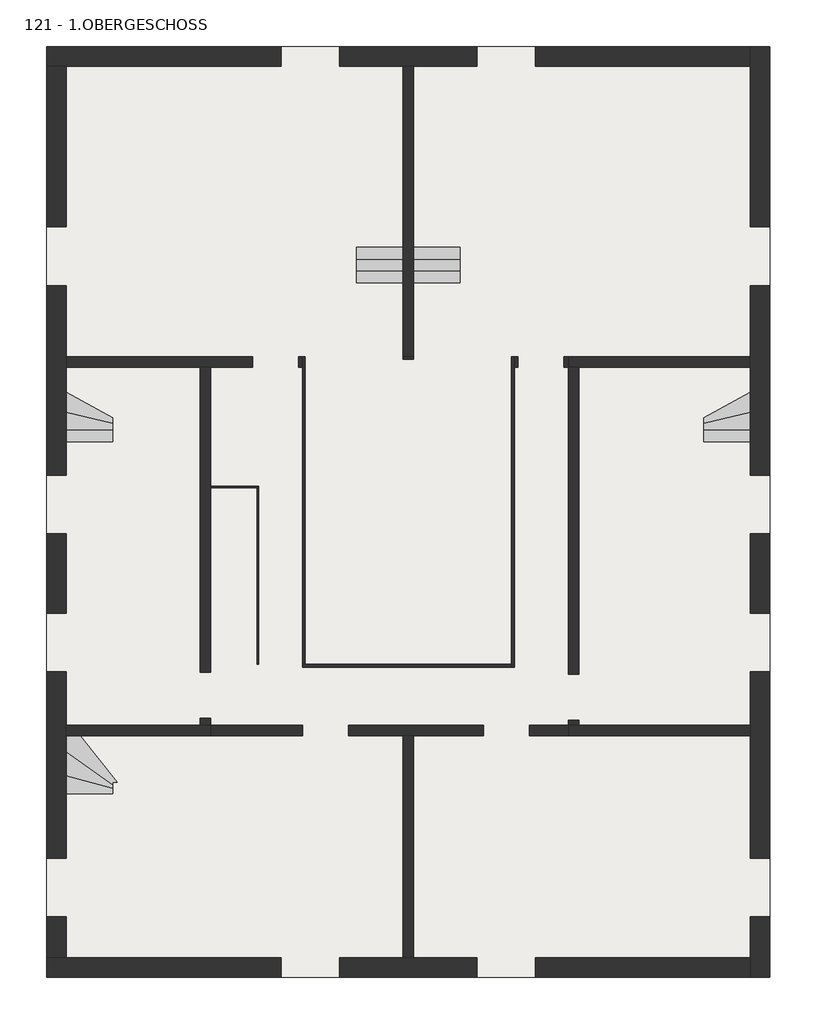
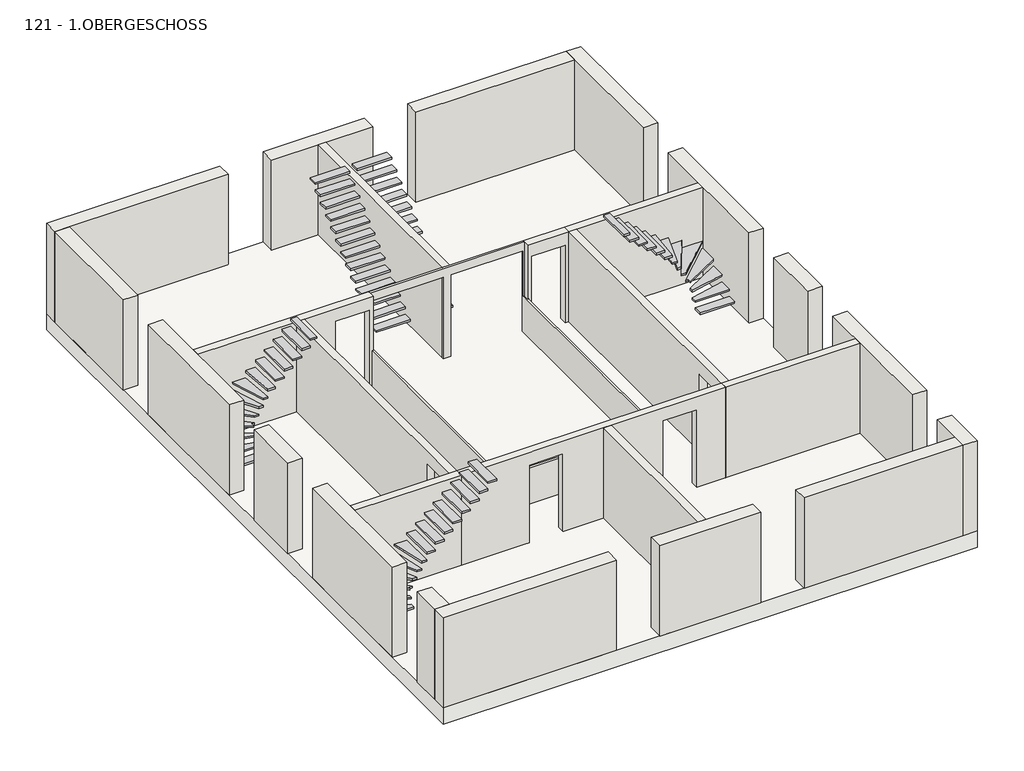
# One storey: 20 walls, 10 stairs, 1 slab.
# Revit data of these elements (continued)
# Type "  98300 :   98300"
#   Abrechnungsart = "St"
#   Allright_Bauteil_ID = "0121Tre0785065278"
#   Codetext = "TR-MASSIV-GER\\"
#   Material = "Stahlbeton"
#   Objektname = "Treppe"
#   NameOverride = " "
#   Reference = "STB-Treppe"
#   ThermalTransmittance = 0.0000 BTU/(h·ft²·°F)
#   NosingLength = 0.000 m
#   NumberOfRiser = 14
#   NumberOfTreads = 13
#   RiserHeight = 2.021 m
#   TreadLength = 2.300 m
#   IsExternal = no
#   FireExit = no
#   HandicapAccessible = no
#   HasNonSkidSurface = no
# Type "  98728 :   98728"
#   Abrechnungsart = "St"
#   Allright_Bauteil_ID = "0121Tre0785070507"
#   Material = "Stahlbeton"
#   Objektname = "Treppe"
#   NameOverride = " "
#   ThermalTransmittance = 0.0000 BTU/(h·ft²·°F)
#   NosingLength = 0.000 m
#   NumberOfRiser = 14
#   NumberOfTreads = 13
#   RiserHeight = 2.021 m
#   TreadLength = 2.300 m
#   IsExternal = no
#   FireExit = no
#   HandicapAccessible = no
#   HasNonSkidSurface = no
# Type "  99154 :   99154"
#   Abrechnungsart = "St"
#   Allright_Bauteil_ID = "0121Tre0785070829"
#   Material = "Stahlbeton"
#   Objektname = "Treppe"
#   NameOverride = " "
#   ThermalTransmittance = 0.0000 BTU/(h·ft²·°F)
#   NosingLength = 0.000 m
#   NumberOfRiser = 14
#   NumberOfTreads = 13
#   RiserHeight = 2.021 m
#   TreadLength = 2.300 m
#   IsExternal = no
#   FireExit = no
#   HandicapAccessible = no
#   HasNonSkidSurface = no
# Type "  149542 :   149542"
#   Abrechnungsart = "St"
#   Allright_Bauteil_ID = "0131Tre0659044515"
#   Material = "Stahlbeton"
#   Objektname = "Treppe"
#   NameOverride = " "
#   ThermalTransmittance = 0.0000 BTU/(h·ft²·°F)
#   NosingLength = 0.000 m
#   NumberOfRiser = 14
#   NumberOfTreads = 14
#   RiserHeight = 2.000 m
#   TreadLength = 2.300 m
#   IsExternal = no
#   FireExit = no
#   HandicapAccessible = no
#   HasNonSkidSurface = no
# Type "  150414 :   150414"
#   Abrechnungsart = "St"
#   Allright_Bauteil_ID = "0131Tre0659044575"
#   Codetext = "TR-MASSIV-GER\\"
#   Material = "Stahlbeton"
#   Objektname = "Treppe"
#   NameOverride = " "
#   Reference = "STB-Treppe"
#   ThermalTransmittance = 0.0000 BTU/(h·ft²·°F)
#   NosingLength = 0.000 m
#   NumberOfRiser = 14
#   NumberOfTreads = 13
#   RiserHeight = 2.021 m
#   TreadLength = 2.300 m
#   IsExternal = no
#   FireExit = no
#   HandicapAccessible = no
#   HasNonSkidSurface = no
# Type "  150832 :   150832"
#   Abrechnungsart = "St"
#   Allright_Bauteil_ID = "0131Tre0659044593"
#   Codetext = "TR-MASSIV-GER\\"
#   Material = "Stahlbeton"
#   Objektname = "Treppe"
#   NameOverride = " "
#   Reference = "STB-Treppe"
#   ThermalTransmittance = 0.0000 BTU/(h·ft²·°F)
#   NosingLength = 0.000 m
#   NumberOfRiser = 14
#   NumberOfTreads = 13
#   RiserHeight = 2.021 m
#   TreadLength = 2.300 m
#   IsExternal = no
#   FireExit = no
#   HandicapAccessible = no
#   HasNonSkidSurface = no
# Type "  151260 :   151260"
#   Abrechnungsart = "St"
#   Allright_Bauteil_ID = "0131Tre0659044533"
#   Material = "Stahlbeton"
#   Objektname = "Treppe"
#   NameOverride = " "
#   ThermalTransmittance = 0.0000 BTU/(h·ft²·°F)
#   NosingLength = 0.000 m
#   NumberOfRiser = 14
#   NumberOfTreads = 13
#   RiserHeight = 2.021 m
#   TreadLength = 2.300 m
#   IsExternal = no
#   FireExit = no
#   HandicapAccessible = no
#   HasNonSkidSurface = no
# Type "  151686 :   151686"
#   Abrechnungsart = "St"
#   Allright_Bauteil_ID = "0131Tre0659044570"
#   Material = "Stahlbeton"
#   Objektname = "Treppe"
#   NameOverride = " "
#   ThermalTransmittance = 0.0000 BTU/(h·ft²·°F)
#   NosingLength = 0.000 m
#   NumberOfRiser = 14
#   NumberOfTreads = 13
#   RiserHeight = 2.021 m
#   TreadLength = 2.300 m
#   IsExternal = no
#   FireExit = no
#   HandicapAccessible = no
#   HasNonSkidSurface = no
# Type " :1166"
#   Layers, outside or top first: 0.050 m "glas" (function 1)
# Type "Holzwand:1150"
#   ThermalTransmittance = 0.0000 BTU/(h·ft²·°F)
#   Combustible = no
#   Compartmentation = no
#   Layers, outside or top first: 0.200 m "holzschalung" (function 1)
# Type "Holzwand:1151"
#   ThermalTransmittance = 0.0000 BTU/(h·ft²·°F)
#   Combustible = no
#   Compartmentation = no
#   Layers, outside or top first: 0.200 m "holzschalung" (function 1)
# Type "Holzwand:1153"
#   ThermalTransmittance = 0.0000 BTU/(h·ft²·°F)
#   Combustible = no
#   Compartmentation = no
#   Layers, outside or top first: 0.200 m "holzschalung" (function 1)
# Type "Holzwand:1154"
#   ThermalTransmittance = 0.0000 BTU/(h·ft²·°F)
#   Combustible = no
#   Compartmentation = no
#   Layers, outside or top first: 0.030 m "holzschalung" (function 1)
# Type "Holzwand:1155"
#   ThermalTransmittance = 0.0000 BTU/(h·ft²·°F)
#   Combustible = no
#   Compartmentation = no
#   Layers, outside or top first: 0.030 m "holzschalung" (function 1)
# Type "Holzwand:1156"
#   ThermalTransmittance = 0.0000 BTU/(h·ft²·°F)
#   Combustible = no
#   Compartmentation = no
#   Layers, outside or top first: 0.200 m "holzschalung" (function 1)
# Type "Holzwand:1157"
#   ThermalTransmittance = 0.0000 BTU/(h·ft²·°F)
#   Combustible = no
#   Compartmentation = no
#   Layers, outside or top first: 0.200 m "holzschalung" (function 1)
# Type "Holzwand:1158"
#   ThermalTransmittance = 0.0000 BTU/(h·ft²·°F)
#   Combustible = no
#   Compartmentation = no
#   Layers, outside or top first: 0.200 m "holzschalung" (function 1)
# Type "Holzwand:1159"
#   ThermalTransmittance = 0.0000 BTU/(h·ft²·°F)
#   Combustible = no
#   Compartmentation = no
#   Layers, outside or top first: 0.200 m "holzschalung" (function 1)
# Type "Holzwand:1160"
#   ThermalTransmittance = 0.0000 BTU/(h·ft²·°F)
#   Combustible = no
#   Compartmentation = no
#   Layers, outside or top first: 0.200 m "holzschalung" (function 1)
# Type "Holzwand:1162"
#   ThermalTransmittance = 0.0000 BTU/(h·ft²·°F)
#   Combustible = no
#   Compartmentation = no
#   Layers, outside or top first: 0.200 m "holzschalung" (function 1)
# Type "Holzwand:1163"
#   ThermalTransmittance = 0.0000 BTU/(h·ft²·°F)
#   Combustible = no
#   Compartmentation = no
#   Layers, outside or top first: 0.200 m "holzschalung" (function 1)
# Type " :1167"
#   Layers, outside or top first: 0.050 m "holzschalung" (function 1)
# Type " :1168"
#   Layers, outside or top first: 0.050 m "holzschalung" (function 1)
# Type " :1169"
#   Layers, outside or top first: 0.050 m "holzschalung" (function 1)
# Type "1141 Aussenwand"
#   Layers, outside or top first: 0.380 m "holzschalung" (function 1)
# Element 1 (IfcSlab, "Holzdecke 176 : Holzdecke 176")
#   IFC Predefined Type = "FLOOR"
#   Export to IFC As = "ifcslab"
#   IfcGUID = "1_9Us2eVX4OuIZjhNyqdxW"
#   Phase Created = New Construction
#   Materials on its faces: "holzschalung"
# Element 2 (IfcStair, "  97010 :   97010")
#   IFC Predefined Type = "NOTDEFINED"
#   Export to IFC As = "ifcstair"
#   IfcGUID = "2ccaodaeb6QgHPV1d4NBnA"
#   Phase Created = New Construction
#   Materials on its faces: "weiss"
# Element 3 (IfcStair, "  97882 :   97882")
#   IFC Predefined Type = "STRAIGHT_RUN_STAIR"
#   Export to IFC As = "ifcstair"
#   IfcGUID = "1nghyUHoH9yBc_lxkBTUjw"
#   Phase Created = New Construction
#   Materials on its faces: "weiss"
# Element 4 (IfcStair, "  98300 :   98300")
#   IFC Predefined Type = "STRAIGHT_RUN_STAIR"
#   Export to IFC As = "ifcstair"
#   IfcGUID = "2AC_Gmfhz1LvYwUyPOxWan"
#   Phase Created = New Construction
#   Materials on its faces: "weiss"
# Element 5 (IfcStair, "  98728 :   98728")
#   IFC Predefined Type = "NOTDEFINED"
#   Export to IFC As = "ifcstair"
#   IfcGUID = "04Edcgbk9CPwWYiYhycXFf"
#   Phase Created = New Construction
#   Materials on its faces: "weiss"
# Element 6 (IfcStair, "  99154 :   99154")
#   IFC Predefined Type = "NOTDEFINED"
#   Export to IFC As = "ifcstair"
#   IfcGUID = "1azVXxNdn2POY9VYN93ccY"
#   Phase Created = New Construction
#   Materials on its faces: "weiss"
# Element 7 (IfcStair, "  149542 :   149542")
#   IFC Predefined Type = "NOTDEFINED"
#   Export to IFC As = "ifcstair"
#   IfcGUID = "1sH4rJKnLAFOtHPnXrLkif"
#   Phase Created = New Construction
#   Materials on its faces: "weiss"
# Element 8 (IfcStair, "  150414 :   150414")
#   IFC Predefined Type = "STRAIGHT_RUN_STAIR"
#   Export to IFC As = "ifcstair"
#   IfcGUID = "3fdccs_Mj1YAyFFpBc3gyk"
#   Phase Created = New Construction
#   Materials on its faces: "weiss"
# Element 9 (IfcStair, "  150832 :   150832")
#   IFC Predefined Type = "STRAIGHT_RUN_STAIR"
#   Export to IFC As = "ifcstair"
#   IfcGUID = "2szmEZdbD3KBDvfX1Sa6Vh"
#   Phase Created = New Construction
#   Materials on its faces: "weiss"
# Element 10 (IfcStair, "  151260 :   151260")
#   IFC Predefined Type = "NOTDEFINED"
#   Export to IFC As = "ifcstair"
#   IfcGUID = "1YKyaFTbr8YR41yGjubBsl"
#   Phase Created = New Construction
#   Materials on its faces: "weiss"
# Element 11 (IfcStair, "  151686 :   151686")
#   IFC Predefined Type = "NOTDEFINED"
#   Export to IFC As = "ifcstair"
#   IfcGUID = "2KPGRYHzzCygzBebAeLtPz"
#   Phase Created = New Construction
#   Materials on its faces: "weiss"
# Element 12 (IfcWall, " :1166")
#   Export to IFC As = "ifcwall"
#   IfcGUID = "0t2qqx1kvDZPNPdKl4bfzP"
#   NameOverride = " "
#   Abrechnungsart = "m³"
#   Allright_Bauteil_ID = "0121HWa0785064296"
#   Layer #1:Object Layer Attributes #1:Abrechnungsart = "m²"
#   Layer #1:Object Layer Attributes #1:Allright_Bauteil_ID = "0121Wa 0785064386"
#   Layer #1:Object Layer Attributes #1:Gewerk = "Zimmer- und Holzbauarbeiten"
#   Layer #1:Object Layer Attributes #1:Material = "k.Ausw."
#   Layer #1:Object Layer Attributes #1:Objektname = "Wand"
#   Layer #1:Object Layer Attributes #1:Status = "Neubau"
#   MEP Wandtyp = "HO-WA-HSW\\"
#   Objektname = "Gesamtwand"
#   built-in parameter 1001111 = 0.505 m
#   Top Offset = 0.000 m
#   Base Offset = 0.505 m
#   Unconnected Height = 2.500 m
#   wall height = 2.500 m
#   Layer #1:Object Layer Attributes #1:2D Interaktion = yes
#   Phase Created = New Construction
#   Base Constraint = 121 - 1.OBERGESCHOSS
#   Materials on its faces: "glas"
# Element 13 (IfcWall, "Holzwand:1150")
#   Export to IFC As = "ifcwall"
#   IfcGUID = "3nZ5Mon9nBjwoRgvyoor9a"
#   NameOverride = "Holzwand"
#   Abrechnungsart = "St"
#   Allright_Bauteil_ID = "0121HWa0785065367"
#   Bezeichnung = "Holzwand"
#   Layer #1:Object Layer Attributes #1:Abrechnungsart = "m²"
#   Layer #1:Object Layer Attributes #1:Allright_Bauteil_ID = "0121Wa 0785065369"
#   Layer #1:Object Layer Attributes #1:Bezeichnung = "Holzwand"
#   Layer #1:Object Layer Attributes #1:Codetext = "HO-WI-HSW\\"
#   Layer #1:Object Layer Attributes #1:Gewerk = "Zimmer- und Holzbauarbeiten"
#   Layer #1:Object Layer Attributes #1:Material = "Holz"
#   Layer #1:Object Layer Attributes #1:Objektname = "Wand"
#   Layer #1:Object Layer Attributes #1:Reference = "Holzwand"
#   Layer #1:Object Layer Attributes #1:Status = "Neubau"
#   MEP Wandtyp = "HO-WA-HSW\\"
#   Objektname = "Gesamtwand"
#   Reference = "Holzwand"
#   Status = "NEW"
#   built-in parameter 1001111 = 0.505 m
#   Top Offset = 0.000 m
#   Base Offset = 0.505 m
#   Unconnected Height = 2.500 m
#   wall height = 2.500 m
#   Layer #1:Object Layer Attributes #1:U-Wert = 0
#   Layer #1:Object Layer Attributes #1:2D Interaktion = yes
#   Layer #1:Object Layer Attributes #1:Außenbauteil = no
#   Layer #1:Object Layer Attributes #1:Brandabschnittsdefinierendes Bauteil = no
#   Layer #1:Object Layer Attributes #1:Brennbares Material = no
#   Layer #1:Object Layer Attributes #1:Raumhohe Wand = yes
#   Layer #1:Object Layer Attributes #1:Tragendes Bauteil = yes
#   ExtendToStructure = yes
#   IsExternal = no
#   LoadBearing = yes
#   Phase Created = New Construction
#   Base Constraint = 121 - 1.OBERGESCHOSS
#   Materials on its faces: "holzschalung"
# Element 14 (IfcWall, "Holzwand:1151")
#   Export to IFC As = "ifcwall"
#   IfcGUID = "3jE1E$NFj7vAP$vn70kdrt"
#   NameOverride = "Holzwand"
#   Abrechnungsart = "St"
#   Allright_Bauteil_ID = "0121HWa0785066899"
#   Bezeichnung = "Holzwand"
#   Layer #1:Object Layer Attributes #1:Abrechnungsart = "m²"
#   Layer #1:Object Layer Attributes #1:Allright_Bauteil_ID = "0121Wa 0785066901"
#   Layer #1:Object Layer Attributes #1:Bezeichnung = "Holzwand"
#   Layer #1:Object Layer Attributes #1:Codetext = "HO-WI-HSW\\"
#   Layer #1:Object Layer Attributes #1:Gewerk = "Zimmer- und Holzbauarbeiten"
#   Layer #1:Object Layer Attributes #1:Material = "Holz"
#   Layer #1:Object Layer Attributes #1:Objektname = "Wand"
#   Layer #1:Object Layer Attributes #1:Reference = "Holzwand"
#   Layer #1:Object Layer Attributes #1:Status = "Neubau"
#   MEP Wandtyp = "HO-WA-HSW\\"
#   Objektname = "Gesamtwand"
#   Reference = "Holzwand"
#   Status = "NEW"
#   built-in parameter 1001111 = 0.505 m
#   Top Offset = 0.000 m
#   Base Offset = 0.505 m
#   Unconnected Height = 2.500 m
#   wall height = 2.500 m
#   Layer #1:Object Layer Attributes #1:U-Wert = 0
#   Layer #1:Object Layer Attributes #1:2D Interaktion = yes
#   Layer #1:Object Layer Attributes #1:Außenbauteil = no
#   Layer #1:Object Layer Attributes #1:Brandabschnittsdefinierendes Bauteil = no
#   Layer #1:Object Layer Attributes #1:Brennbares Material = no
#   Layer #1:Object Layer Attributes #1:Raumhohe Wand = yes
#   Layer #1:Object Layer Attributes #1:Tragendes Bauteil = yes
#   ExtendToStructure = yes
#   IsExternal = no
#   LoadBearing = yes
#   Phase Created = New Construction
#   Base Constraint = 121 - 1.OBERGESCHOSS
#   Materials on its faces: "holzschalung"
# Element 15 (IfcWall, "Holzwand:1153")
#   Export to IFC As = "ifcwall"
#   IfcGUID = "1Zhxv5EALB9e6_$pCtUEXg"
#   NameOverride = "Holzwand"
#   Abrechnungsart = "St"
#   Allright_Bauteil_ID = "0121HWa0785065540"
#   Bezeichnung = "Holzwand"
#   Layer #1:Object Layer Attributes #1:Abrechnungsart = "m²"
#   Layer #1:Object Layer Attributes #1:Allright_Bauteil_ID = "0121Wa 0785065541"
#   Layer #1:Object Layer Attributes #1:Bezeichnung = "Holzwand"
#   Layer #1:Object Layer Attributes #1:Codetext = "HO-WI-HSW\\"
#   Layer #1:Object Layer Attributes #1:Gewerk = "Zimmer- und Holzbauarbeiten"
#   Layer #1:Object Layer Attributes #1:Material = "Holz"
#   Layer #1:Object Layer Attributes #1:Objektname = "Wand"
#   Layer #1:Object Layer Attributes #1:Reference = "Holzwand"
#   Layer #1:Object Layer Attributes #1:Status = "Neubau"
#   MEP Wandtyp = "HO-WA-HSW\\"
#   Objektname = "Gesamtwand"
#   Reference = "Holzwand"
#   Status = "NEW"
#   built-in parameter 1001111 = 0.505 m
#   Top Offset = 0.000 m
#   Base Offset = 0.505 m
#   Unconnected Height = 2.500 m
#   wall height = 2.500 m
#   Layer #1:Object Layer Attributes #1:U-Wert = 0
#   Layer #1:Object Layer Attributes #1:2D Interaktion = yes
#   Layer #1:Object Layer Attributes #1:Außenbauteil = no
#   Layer #1:Object Layer Attributes #1:Brandabschnittsdefinierendes Bauteil = no
#   Layer #1:Object Layer Attributes #1:Brennbares Material = no
#   Layer #1:Object Layer Attributes #1:Raumhohe Wand = yes
#   Layer #1:Object Layer Attributes #1:Tragendes Bauteil = yes
#   ExtendToStructure = yes
#   IsExternal = no
#   LoadBearing = yes
#   Phase Created = New Construction
#   Base Constraint = 121 - 1.OBERGESCHOSS
#   Materials on its faces: "holzschalung"
# Element 16 (IfcWall, "Holzwand:1154")
#   Export to IFC As = "ifcwall"
#   IfcGUID = "2MsVq3EJn0K8wHdQ6uoxnd"
#   NameOverride = "Holzwand"
#   Abrechnungsart = "St"
#   Allright_Bauteil_ID = "0121HWa0785067355"
#   Bezeichnung = "Holzwand"
#   Layer #1:Object Layer Attributes #1:Abrechnungsart = "m²"
#   Layer #1:Object Layer Attributes #1:Allright_Bauteil_ID = "0121Wa 0785067356"
#   Layer #1:Object Layer Attributes #1:Codetext = "HO-WI-HSW\\"
#   Layer #1:Object Layer Attributes #1:Gewerk = "Zimmer- und Holzbauarbeiten"
#   Layer #1:Object Layer Attributes #1:Material = "Holz"
#   Layer #1:Object Layer Attributes #1:Objektname = "Wand"
#   Layer #1:Object Layer Attributes #1:Reference = "Holzwand"
#   Layer #1:Object Layer Attributes #1:Status = "Neubau"
#   MEP Wandtyp = "HO-WA-HSW\\"
#   Objektname = "Gesamtwand"
#   Reference = "Holzwand"
#   Status = "NEW"
#   built-in parameter 1001111 = 0.505 m
#   Top Offset = 0.000 m
#   Base Offset = 0.505 m
#   Unconnected Height = 1.000 m
#   wall height = 1.000 m
#   Layer #1:Object Layer Attributes #1:U-Wert = 0
#   Layer #1:Object Layer Attributes #1:2D Interaktion = yes
#   Layer #1:Object Layer Attributes #1:Außenbauteil = no
#   Layer #1:Object Layer Attributes #1:Brandabschnittsdefinierendes Bauteil = no
#   Layer #1:Object Layer Attributes #1:Brennbares Material = no
#   Layer #1:Object Layer Attributes #1:Raumhohe Wand = yes
#   ExtendToStructure = yes
#   IsExternal = no
#   LoadBearing = yes
#   Phase Created = New Construction
#   Base Constraint = 121 - 1.OBERGESCHOSS
#   Materials on its faces: "holzschalung"
# Element 17 (IfcWall, "Holzwand:1155")
#   Export to IFC As = "ifcwall"
#   IfcGUID = "1F_ySrDsP9oP3MqXymSTVO"
#   NameOverride = "Holzwand"
#   Abrechnungsart = "St"
#   Allright_Bauteil_ID = "0121HWa0785067347"
#   Bezeichnung = "Holzwand"
#   Layer #1:Object Layer Attributes #1:Abrechnungsart = "m²"
#   Layer #1:Object Layer Attributes #1:Allright_Bauteil_ID = "0121Wa 0785067348"
#   Layer #1:Object Layer Attributes #1:Codetext = "HO-WI-HSW\\"
#   Layer #1:Object Layer Attributes #1:Gewerk = "Zimmer- und Holzbauarbeiten"
#   Layer #1:Object Layer Attributes #1:Material = "Holz"
#   Layer #1:Object Layer Attributes #1:Objektname = "Wand"
#   Layer #1:Object Layer Attributes #1:Reference = "Holzwand"
#   Layer #1:Object Layer Attributes #1:Status = "Neubau"
#   MEP Wandtyp = "HO-WA-HSW\\"
#   Objektname = "Gesamtwand"
#   Reference = "Holzwand"
#   Status = "NEW"
#   built-in parameter 1001111 = 0.505 m
#   Top Offset = 0.000 m
#   Base Offset = 0.505 m
#   Unconnected Height = 1.000 m
#   wall height = 1.000 m
#   Layer #1:Object Layer Attributes #1:U-Wert = 0
#   Layer #1:Object Layer Attributes #1:2D Interaktion = yes
#   Layer #1:Object Layer Attributes #1:Außenbauteil = no
#   Layer #1:Object Layer Attributes #1:Brandabschnittsdefinierendes Bauteil = no
#   Layer #1:Object Layer Attributes #1:Brennbares Material = no
#   Layer #1:Object Layer Attributes #1:Raumhohe Wand = yes
#   ExtendToStructure = yes
#   IsExternal = no
#   LoadBearing = yes
#   Phase Created = New Construction
#   Base Constraint = 121 - 1.OBERGESCHOSS
#   Materials on its faces: "holzschalung"
# Element 18 (IfcWall, "Holzwand:1156")
#   Export to IFC As = "ifcwall"
#   IfcGUID = "0gtwZwppj1pObqyI7HY41_"
#   NameOverride = "Holzwand"
#   Abrechnungsart = "St"
#   Allright_Bauteil_ID = "0121HWa0785064323"
#   Bezeichnung = "Holzwand"
#   Layer #1:Object Layer Attributes #1:Abrechnungsart = "m²"
#   Layer #1:Object Layer Attributes #1:Allright_Bauteil_ID = "0121Wa 0785064369"
#   Layer #1:Object Layer Attributes #1:Bezeichnung = "Holzwand"
#   Layer #1:Object Layer Attributes #1:Codetext = "HO-WI-HSW\\"
#   Layer #1:Object Layer Attributes #1:Gewerk = "Zimmer- und Holzbauarbeiten"
#   Layer #1:Object Layer Attributes #1:Material = "Holz"
#   Layer #1:Object Layer Attributes #1:Objektname = "Wand"
#   Layer #1:Object Layer Attributes #1:Reference = "Holzwand"
#   Layer #1:Object Layer Attributes #1:Status = "Neubau"
#   MEP Wandtyp = "HO-WA-HSW\\"
#   Objektname = "Gesamtwand"
#   Reference = "Holzwand"
#   Status = "NEW"
#   built-in parameter 1001111 = 0.505 m
#   Top Offset = 0.000 m
#   Base Offset = 0.505 m
#   Unconnected Height = 2.500 m
#   wall height = 2.500 m
#   Layer #1:Object Layer Attributes #1:U-Wert = 0
#   Layer #1:Object Layer Attributes #1:2D Interaktion = yes
#   Layer #1:Object Layer Attributes #1:Außenbauteil = no
#   Layer #1:Object Layer Attributes #1:Brandabschnittsdefinierendes Bauteil = no
#   Layer #1:Object Layer Attributes #1:Brennbares Material = no
#   Layer #1:Object Layer Attributes #1:Raumhohe Wand = yes
#   Layer #1:Object Layer Attributes #1:Tragendes Bauteil = yes
#   ExtendToStructure = yes
#   IsExternal = no
#   LoadBearing = yes
#   Phase Created = New Construction
#   Base Constraint = 121 - 1.OBERGESCHOSS
#   Materials on its faces: "holzschalung"
# Element 19 (IfcWall, "Holzwand:1157")
#   Export to IFC As = "ifcwall"
#   IfcGUID = "0tY6$O1l121AktLhYSWZjf"
#   NameOverride = "Holzwand"
#   Abrechnungsart = "St"
#   Allright_Bauteil_ID = "0121HWa0785064381"
#   Bezeichnung = "Holzwand"
#   Layer #1:Object Layer Attributes #1:Abrechnungsart = "m²"
#   Layer #1:Object Layer Attributes #1:Allright_Bauteil_ID = "0121Wa 0785064384"
#   Layer #1:Object Layer Attributes #1:Bezeichnung = "Holzwand"
#   Layer #1:Object Layer Attributes #1:Codetext = "HO-WI-HSW\\"
#   Layer #1:Object Layer Attributes #1:Gewerk = "Zimmer- und Holzbauarbeiten"
#   Layer #1:Object Layer Attributes #1:Material = "Holz"
#   Layer #1:Object Layer Attributes #1:Objektname = "Wand"
#   Layer #1:Object Layer Attributes #1:Reference = "Holzwand"
#   Layer #1:Object Layer Attributes #1:Status = "Neubau"
#   MEP Wandtyp = "HO-WA-HSW\\"
#   Objektname = "Gesamtwand"
#   Reference = "Holzwand"
#   Status = "NEW"
#   built-in parameter 1001111 = 0.505 m
#   Top Offset = 0.000 m
#   Base Offset = 0.505 m
#   Unconnected Height = 2.500 m
#   wall height = 2.500 m
#   Layer #1:Object Layer Attributes #1:U-Wert = 0
#   Layer #1:Object Layer Attributes #1:2D Interaktion = yes
#   Layer #1:Object Layer Attributes #1:Außenbauteil = no
#   Layer #1:Object Layer Attributes #1:Brandabschnittsdefinierendes Bauteil = no
#   Layer #1:Object Layer Attributes #1:Brennbares Material = no
#   Layer #1:Object Layer Attributes #1:Raumhohe Wand = yes
#   Layer #1:Object Layer Attributes #1:Tragendes Bauteil = yes
#   ExtendToStructure = yes
#   IsExternal = no
#   LoadBearing = yes
#   Phase Created = New Construction
#   Base Constraint = 121 - 1.OBERGESCHOSS
#   Materials on its faces: "holzschalung"
# Element 20 (IfcWall, "Holzwand:1158")
#   Export to IFC As = "ifcwall"
#   IfcGUID = "2Mr8L52dj4iP8MoJTiOa9p"
#   NameOverride = "Holzwand"
#   Abrechnungsart = "St"
#   Allright_Bauteil_ID = "0121HWa0785069286"
#   Bezeichnung = "Holzwand"
#   Layer #1:Object Layer Attributes #1:Abrechnungsart = "m²"
#   Layer #1:Object Layer Attributes #1:Allright_Bauteil_ID = "0121Wa 0785069294"
#   Layer #1:Object Layer Attributes #1:Bezeichnung = "Holzwand"
#   Layer #1:Object Layer Attributes #1:Codetext = "HO-WI-HSW\\"
#   Layer #1:Object Layer Attributes #1:Gewerk = "Zimmer- und Holzbauarbeiten"
#   Layer #1:Object Layer Attributes #1:Material = "Holz"
#   Layer #1:Object Layer Attributes #1:Objektname = "Wand"
#   Layer #1:Object Layer Attributes #1:Reference = "Holzwand"
#   Layer #1:Object Layer Attributes #1:Status = "Neubau"
#   MEP Wandtyp = "HO-WA-HSW\\"
#   Objektname = "Gesamtwand"
#   Reference = "Holzwand"
#   Status = "NEW"
#   built-in parameter 1001111 = 0.505 m
#   Top Offset = 0.000 m
#   Base Offset = 0.505 m
#   Unconnected Height = 2.500 m
#   wall height = 2.500 m
#   Layer #1:Object Layer Attributes #1:U-Wert = 0
#   Layer #1:Object Layer Attributes #1:2D Interaktion = yes
#   Layer #1:Object Layer Attributes #1:Außenbauteil = no
#   Layer #1:Object Layer Attributes #1:Brandabschnittsdefinierendes Bauteil = no
#   Layer #1:Object Layer Attributes #1:Brennbares Material = no
#   Layer #1:Object Layer Attributes #1:Raumhohe Wand = yes
#   Layer #1:Object Layer Attributes #1:Tragendes Bauteil = yes
#   ExtendToStructure = yes
#   IsExternal = no
#   LoadBearing = yes
#   Phase Created = New Construction
#   Base Constraint = 121 - 1.OBERGESCHOSS
#   Materials on its faces: "holzschalung"
# Element 21 (IfcWall, "Holzwand:1159")
#   Export to IFC As = "ifcwall"
#   IfcGUID = "36leNf4gL9OB_v358ffY76"
#   NameOverride = "Holzwand"
#   Abrechnungsart = "St"
#   Allright_Bauteil_ID = "0121HWa0785064324"
#   Bezeichnung = "Holzwand"
#   Layer #1:Object Layer Attributes #1:Abrechnungsart = "m²"
#   Layer #1:Object Layer Attributes #1:Allright_Bauteil_ID = "0121Wa 0785064395"
#   Layer #1:Object Layer Attributes #1:Bezeichnung = "Holzwand"
#   Layer #1:Object Layer Attributes #1:Codetext = "HO-WI-HSW\\"
#   Layer #1:Object Layer Attributes #1:Gewerk = "Zimmer- und Holzbauarbeiten"
#   Layer #1:Object Layer Attributes #1:Material = "Holz"
#   Layer #1:Object Layer Attributes #1:Objektname = "Wand"
#   Layer #1:Object Layer Attributes #1:Reference = "Holzwand"
#   Layer #1:Object Layer Attributes #1:Status = "Neubau"
#   MEP Wandtyp = "HO-WA-HSW\\"
#   Objektname = "Gesamtwand"
#   Reference = "Holzwand"
#   Status = "NEW"
#   built-in parameter 1001111 = 0.505 m
#   Top Offset = 0.000 m
#   Base Offset = 0.505 m
#   Unconnected Height = 2.500 m
#   wall height = 2.500 m
#   Layer #1:Object Layer Attributes #1:U-Wert = 0
#   Layer #1:Object Layer Attributes #1:2D Interaktion = yes
#   Layer #1:Object Layer Attributes #1:Außenbauteil = no
#   Layer #1:Object Layer Attributes #1:Brandabschnittsdefinierendes Bauteil = no
#   Layer #1:Object Layer Attributes #1:Brennbares Material = no
#   Layer #1:Object Layer Attributes #1:Raumhohe Wand = yes
#   Layer #1:Object Layer Attributes #1:Tragendes Bauteil = yes
#   ExtendToStructure = yes
#   IsExternal = no
#   LoadBearing = yes
#   Phase Created = New Construction
#   Base Constraint = 121 - 1.OBERGESCHOSS
#   Materials on its faces: "holzschalung"
# Element 22 (IfcWall, "Holzwand:1160")
#   Export to IFC As = "ifcwall"
#   IfcGUID = "3kHHpx_NTE_9JnfL3dFkYB"
#   NameOverride = "Holzwand"
#   Abrechnungsart = "St"
#   Allright_Bauteil_ID = "0121HWa0785064389"
#   Bezeichnung = "Holzwand"
#   Layer #1:Object Layer Attributes #1:Abrechnungsart = "m²"
#   Layer #1:Object Layer Attributes #1:Allright_Bauteil_ID = "0121Wa 0785064393"
#   Layer #1:Object Layer Attributes #1:Bezeichnung = "Holzwand"
#   Layer #1:Object Layer Attributes #1:Codetext = "HO-WI-HSW\\"
#   Layer #1:Object Layer Attributes #1:Gewerk = "Zimmer- und Holzbauarbeiten"
#   Layer #1:Object Layer Attributes #1:Material = "Holz"
#   Layer #1:Object Layer Attributes #1:Objektname = "Wand"
#   Layer #1:Object Layer Attributes #1:Reference = "Holzwand"
#   Layer #1:Object Layer Attributes #1:Status = "Neubau"
#   MEP Wandtyp = "HO-WA-HSW\\"
#   Objektname = "Gesamtwand"
#   Reference = "Holzwand"
#   Status = "NEW"
#   built-in parameter 1001111 = 0.505 m
#   Top Offset = 0.000 m
#   Base Offset = 0.505 m
#   Unconnected Height = 2.500 m
#   wall height = 2.500 m
#   Layer #1:Object Layer Attributes #1:U-Wert = 0
#   Layer #1:Object Layer Attributes #1:2D Interaktion = yes
#   Layer #1:Object Layer Attributes #1:Außenbauteil = no
#   Layer #1:Object Layer Attributes #1:Brandabschnittsdefinierendes Bauteil = no
#   Layer #1:Object Layer Attributes #1:Brennbares Material = no
#   Layer #1:Object Layer Attributes #1:Raumhohe Wand = yes
#   Layer #1:Object Layer Attributes #1:Tragendes Bauteil = yes
#   ExtendToStructure = yes
#   IsExternal = no
#   LoadBearing = yes
#   Phase Created = New Construction
#   Base Constraint = 121 - 1.OBERGESCHOSS
#   Materials on its faces: "holzschalung"
# Element 23 (IfcWall, "Holzwand:1162")
#   Export to IFC As = "ifcwall"
#   IfcGUID = "26lQuimMP00PZvPhbBRI2R"
#   NameOverride = "Holzwand"
#   Abrechnungsart = "St"
#   Allright_Bauteil_ID = "0121HWa0785065329"
#   Bezeichnung = "Holzwand"
#   Layer #1:Object Layer Attributes #1:Abrechnungsart = "m²"
#   Layer #1:Object Layer Attributes #1:Allright_Bauteil_ID = "0121Wa 0785065331"
#   Layer #1:Object Layer Attributes #1:Bezeichnung = "Holzwand"
#   Layer #1:Object Layer Attributes #1:Codetext = "HO-WI-HSW\\"
#   Layer #1:Object Layer Attributes #1:Gewerk = "Zimmer- und Holzbauarbeiten"
#   Layer #1:Object Layer Attributes #1:Material = "Holz"
#   Layer #1:Object Layer Attributes #1:Objektname = "Wand"
#   Layer #1:Object Layer Attributes #1:Reference = "Holzwand"
#   Layer #1:Object Layer Attributes #1:Status = "Neubau"
#   MEP Wandtyp = "HO-WA-HSW\\"
#   Objektname = "Gesamtwand"
#   Reference = "Holzwand"
#   Status = "NEW"
#   built-in parameter 1001111 = 0.505 m
#   Top Offset = 0.000 m
#   Base Offset = 0.505 m
#   Unconnected Height = 2.500 m
#   wall height = 2.500 m
#   Layer #1:Object Layer Attributes #1:U-Wert = 0
#   Layer #1:Object Layer Attributes #1:2D Interaktion = yes
#   Layer #1:Object Layer Attributes #1:Außenbauteil = no
#   Layer #1:Object Layer Attributes #1:Brandabschnittsdefinierendes Bauteil = no
#   Layer #1:Object Layer Attributes #1:Brennbares Material = no
#   Layer #1:Object Layer Attributes #1:Raumhohe Wand = yes
#   Layer #1:Object Layer Attributes #1:Tragendes Bauteil = yes
#   ExtendToStructure = yes
#   IsExternal = no
#   LoadBearing = yes
#   Phase Created = New Construction
#   Base Constraint = 121 - 1.OBERGESCHOSS
#   Materials on its faces: "holzschalung"
# Element 24 (IfcWall, "Holzwand:1163")
#   Export to IFC As = "ifcwall"
#   IfcGUID = "3atU$IMTH8YP$GZozT8ehc"
#   NameOverride = "Holzwand"
#   Abrechnungsart = "St"
#   Allright_Bauteil_ID = "0121HWa0785064334"
#   Bezeichnung = "Holzwand"
#   Layer #1:Object Layer Attributes #1:Abrechnungsart = "m²"
#   Layer #1:Object Layer Attributes #1:Allright_Bauteil_ID = "0121Wa 0785064371"
#   Layer #1:Object Layer Attributes #1:Bezeichnung = "Holzwand"
#   Layer #1:Object Layer Attributes #1:Codetext = "HO-WI-HSW\\"
#   Layer #1:Object Layer Attributes #1:Gewerk = "Zimmer- und Holzbauarbeiten"
#   Layer #1:Object Layer Attributes #1:Material = "Holz"
#   Layer #1:Object Layer Attributes #1:Objektname = "Wand"
#   Layer #1:Object Layer Attributes #1:Reference = "Holzwand"
#   Layer #1:Object Layer Attributes #1:Status = "Neubau"
#   MEP Wandtyp = "HO-WA-HSW\\"
#   Objektname = "Gesamtwand"
#   Reference = "Holzwand"
#   Status = "NEW"
#   built-in parameter 1001111 = 0.505 m
#   Top Offset = 0.000 m
#   Base Offset = 0.505 m
#   Unconnected Height = 2.500 m
#   wall height = 2.500 m
#   Layer #1:Object Layer Attributes #1:U-Wert = 0
#   Layer #1:Object Layer Attributes #1:2D Interaktion = yes
#   Layer #1:Object Layer Attributes #1:Außenbauteil = no
#   Layer #1:Object Layer Attributes #1:Brandabschnittsdefinierendes Bauteil = no
#   Layer #1:Object Layer Attributes #1:Brennbares Material = no
#   Layer #1:Object Layer Attributes #1:Raumhohe Wand = yes
#   Layer #1:Object Layer Attributes #1:Tragendes Bauteil = yes
#   ExtendToStructure = yes
#   IsExternal = no
#   LoadBearing = yes
#   Phase Created = New Construction
#   Base Constraint = 121 - 1.OBERGESCHOSS
#   Materials on its faces: "holzschalung"
# Element 25 (IfcWall, " :1167")
#   Export to IFC As = "ifcwall"
#   IfcGUID = "35Iolt9MTFw82QPYPk5JvU"
#   NameOverride = " "
#   Abrechnungsart = "m³"
#   Allright_Bauteil_ID = "0121HWa0785064294"
#   Layer #1:Object Layer Attributes #1:Abrechnungsart = "m²"
#   Layer #1:Object Layer Attributes #1:Allright_Bauteil_ID = "0121Wa 0785064340"
#   Layer #1:Object Layer Attributes #1:Gewerk = "Zimmer- und Holzbauarbeiten"
#   Layer #1:Object Layer Attributes #1:Material = "k.Ausw."
#   Layer #1:Object Layer Attributes #1:Objektname = "Wand"
#   Layer #1:Object Layer Attributes #1:Status = "Neubau"
#   MEP Wandtyp = "HO-WA-HSW\\"
#   Objektname = "Gesamtwand"
#   built-in parameter 1001111 = 0.505 m
#   Top Offset = 0.000 m
#   Base Offset = 0.505 m
#   Unconnected Height = 1.000 m
#   wall height = 1.000 m
#   Layer #1:Object Layer Attributes #1:2D Interaktion = yes
#   Layer #1:Object Layer Attributes #1:Tragendes Bauteil = no
#   Phase Created = New Construction
#   Base Constraint = 121 - 1.OBERGESCHOSS
#   Materials on its faces: "holzschalung", "glas"
# Element 26 (IfcWall, " :1168")
#   Export to IFC As = "ifcwall"
#   IfcGUID = "21NDiotIv7sAO2c5Bbio25"
#   NameOverride = " "
#   Abrechnungsart = "m³"
#   Allright_Bauteil_ID = "0121HWa0785064290"
#   Layer #1:Object Layer Attributes #1:Abrechnungsart = "m²"
#   Layer #1:Object Layer Attributes #1:Allright_Bauteil_ID = "0121Wa 0785064348"
#   Layer #1:Object Layer Attributes #1:Gewerk = "Zimmer- und Holzbauarbeiten"
#   Layer #1:Object Layer Attributes #1:Material = "k.Ausw."
#   Layer #1:Object Layer Attributes #1:Objektname = "Wand"
#   Layer #1:Object Layer Attributes #1:Status = "Neubau"
#   MEP Wandtyp = "HO-WA-HSW\\"
#   Objektname = "Gesamtwand"
#   built-in parameter 1001111 = 0.505 m
#   Top Offset = 0.000 m
#   Base Offset = 0.505 m
#   Unconnected Height = 1.000 m
#   wall height = 1.000 m
#   Layer #1:Object Layer Attributes #1:2D Interaktion = yes
#   Layer #1:Object Layer Attributes #1:Tragendes Bauteil = no
#   Phase Created = New Construction
#   Base Constraint = 121 - 1.OBERGESCHOSS
#   Materials on its faces: "holzschalung"
# Element 27 (IfcWall, " :1169")
#   Export to IFC As = "ifcwall"
#   IfcGUID = "2aL_F8tebFMgUeEEKPH5KO"
#   NameOverride = " "
#   Abrechnungsart = "m³"
#   Allright_Bauteil_ID = "0121HWa0785064292"
#   Layer #1:Object Layer Attributes #1:Abrechnungsart = "m²"
#   Layer #1:Object Layer Attributes #1:Allright_Bauteil_ID = "0121Wa 0785064346"
#   Layer #1:Object Layer Attributes #1:Gewerk = "Zimmer- und Holzbauarbeiten"
#   Layer #1:Object Layer Attributes #1:Material = "k.Ausw."
#   Layer #1:Object Layer Attributes #1:Objektname = "Wand"
#   Layer #1:Object Layer Attributes #1:Status = "Neubau"
#   MEP Wandtyp = "HO-WA-HSW\\"
#   Objektname = "Gesamtwand"
#   built-in parameter 1001111 = 0.505 m
#   Top Offset = 0.000 m
#   Base Offset = 0.505 m
#   Unconnected Height = 1.000 m
#   wall height = 1.000 m
#   Layer #1:Object Layer Attributes #1:2D Interaktion = yes
#   Layer #1:Object Layer Attributes #1:Tragendes Bauteil = no
#   Phase Created = New Construction
#   Base Constraint = 121 - 1.OBERGESCHOSS
#   Materials on its faces: "holzschalung", "glas"
# Element 28 (IfcWall, "1141 Aussenwand")
#   Export to IFC As = "ifcwall"
#   IfcGUID = "2CeDj8YZTCPx$yj4WDVOez"
#   NameOverride = " "
#   Abrechnungsart = "m³"
#   Allright_Bauteil_ID = "0121HWa0785064286"
#   Layer #1:Object Layer Attributes #1:Abrechnungsart = "m²"
#   Layer #1:Object Layer Attributes #1:Allright_Bauteil_ID = "0121Wa 0785064367"
#   Layer #1:Object Layer Attributes #1:Gewerk = "Zimmer- und Holzbauarbeiten"
#   Layer #1:Object Layer Attributes #1:Material = "k.Ausw."
#   Layer #1:Object Layer Attributes #1:Objektname = "Wand"
#   Layer #1:Object Layer Attributes #1:Status = "Neubau"
#   MEP Wandtyp = "HO-WA-HSW\\"
#   Objektname = "Gesamtwand"
#   built-in parameter 1001111 = 0.505 m
#   Top Offset = 0.000 m
#   Base Offset = 0.505 m
#   Unconnected Height = 2.500 m
#   wall height = 2.500 m
#   Layer #1:Object Layer Attributes #1:2D Interaktion = yes
#   Phase Created = New Construction
#   Base Constraint = 121 - 1.OBERGESCHOSS
#   Materials on its faces: "holzschalung"
# Element 29 (IfcWall, "1141 Aussenwand")
#   Export to IFC As = "ifcwall"
#   IfcGUID = "2TnImcbz91shb3jN7Wgb8B"
#   Comments = "OG Sued"
#   Mark = "OG Sued"
#   NameOverride = " "
#   Abrechnungsart = "m³"
#   Allright_Bauteil_ID = "0121HWa0785064349"
#   Layer #1:Object Layer Attributes #1:Abrechnungsart = "m²"
#   Layer #1:Object Layer Attributes #1:Allright_Bauteil_ID = "0121Wa 0785064397"
#   Layer #1:Object Layer Attributes #1:Gewerk = "Zimmer- und Holzbauarbeiten"
#   Layer #1:Object Layer Attributes #1:Material = "k.Ausw."
#   Layer #1:Object Layer Attributes #1:Objektname = "Wand"
#   Layer #1:Object Layer Attributes #1:Status = "Neubau"
#   MEP Wandtyp = "HO-WA-HSW\\"
#   Objektname = "Gesamtwand"
#   built-in parameter 1001111 = 0.505 m
#   Top Offset = 0.000 m
#   Base Offset = 0.505 m
#   Unconnected Height = 2.500 m
#   wall height = 2.500 m
#   Layer #1:Object Layer Attributes #1:2D Interaktion = yes
#   Phase Created = New Construction
#   Base Constraint = 121 - 1.OBERGESCHOSS
#   Materials on its faces: "holzschalung"
# Element 30 (IfcWall, "1141 Aussenwand")
#   Export to IFC As = "ifcwall"
#   IfcGUID = "1tWRh4hxLAdASVw4VNE3to"
#   NameOverride = " "
#   Abrechnungsart = "m³"
#   Allright_Bauteil_ID = "0121HWa0785092952"
#   Layer #1:Object Layer Attributes #1:Abrechnungsart = "m²"
#   Layer #1:Object Layer Attributes #1:Allright_Bauteil_ID = "0121Wa 0785092986"
#   Layer #1:Object Layer Attributes #1:Gewerk = "Zimmer- und Holzbauarbeiten"
#   Layer #1:Object Layer Attributes #1:Material = "k.Ausw."
#   Layer #1:Object Layer Attributes #1:Objektname = "Wand"
#   Layer #1:Object Layer Attributes #1:Status = "Neubau"
#   MEP Wandtyp = "HO-WA-HSW\\"
#   Objektname = "Gesamtwand"
#   built-in parameter 1001111 = 0.505 m
#   Top Offset = 0.000 m
#   Base Offset = 0.505 m
#   Unconnected Height = 2.500 m
#   wall height = 2.500 m
#   Layer #1:Object Layer Attributes #1:2D Interaktion = yes
#   Phase Created = New Construction
#   Base Constraint = 121 - 1.OBERGESCHOSS
#   Materials on its faces: "holzschalung"
# Element 31 (IfcWall, "1141 Aussenwand")
#   Export to IFC As = "ifcwall"
#   IfcGUID = "1HE73MTmDEEBf4AV7ughZ8"
#   NameOverride = " "
#   Abrechnungsart = "m³"
#   Allright_Bauteil_ID = "0121HWa0785097898"
#   Layer #1:Object Layer Attributes #1:Abrechnungsart = "m²"
#   Layer #1:Object Layer Attributes #1:Allright_Bauteil_ID = "0121Wa 0785097934"
#   Layer #1:Object Layer Attributes #1:Gewerk = "Zimmer- und Holzbauarbeiten"
#   Layer #1:Object Layer Attributes #1:Material = "k.Ausw."
#   Layer #1:Object Layer Attributes #1:Objektname = "Wand"
#   Layer #1:Object Layer Attributes #1:Status = "Neubau"
#   MEP Wandtyp = "HO-WA-HSW\\"
#   Objektname = "Gesamtwand"
#   built-in parameter 1001111 = 0.505 m
#   Top Offset = 0.000 m
#   Base Offset = 0.505 m
#   Unconnected Height = 2.500 m
#   wall height = 2.500 m
#   Layer #1:Object Layer Attributes #1:2D Interaktion = yes
#   Phase Created = New Construction
#   Base Constraint = 121 - 1.OBERGESCHOSS
#   Materials on its faces: "holzschalung"
# Materials
#   "glas": class "Unassigned", colour RGB 250 253 254, transparency 0.95
#   "holzschalung": class "Unassigned", colour RGB 128 128 128, transparency 0
#   "weiss": class "Unassigned", colour RGB 255 255 255, transparency 0
# Room at (13460, 8317.808) mm, phase "New Construction", upper offset 2.500 m, lower offset 0.000 m
#   Export to IFC As = "ifcspace"
#   IfcGUID = "3ldkF51q96e9r6BFrUoGvb"
#   Comments = ""
#   Number = "30"
#   Name = "Zimmer 4"
#   Abrechnungsart = "m²"
#   Allright_Bauteil_ID = "0121Rau0785070860"
#   Objektname = "Raum"
#   Status = "Neubau"
#   Flächenart_DIN277 = "N"
#   Flächenart_Wohnfläche = "WO"
#   Nutzungsart_Din277 = "NUF"
#   Ortscode_Geschoßbezeichnung = "OG"
#   Raumumschließung = "R"
#   Faktor_DIN277 = 1
#   Faktor_Wohnfläche_Raum = 1
#   BauNVO_Anrechnung_auf_GF = 0
#   BauNVO_Anrechnung_auf_GR = 0
#   Raum unter Treppe (Wohnfl erst ab 2m) = 0
# Room at (3177.5, 8317.808) mm, phase "New Construction", upper offset 2.500 m, lower offset 0.000 m
#   Export to IFC As = "ifcspace"
#   IfcGUID = "0$kYsoxCXA3h__RP_0NR6Q"
#   Comments = ""
#   Number = "31"
#   Name = "Zimmer 7"
#   Abrechnungsart = "m²"
#   Allright_Bauteil_ID = "0121Rau0785070777"
#   Objektname = "Raum"
#   Status = "Neubau"
#   Flächenart_DIN277 = "N"
#   Flächenart_Wohnfläche = "WO"
#   Nutzungsart_Din277 = "NUF"
#   Ortscode_Geschoßbezeichnung = "OG"
#   Raumumschließung = "R"
#   Faktor_DIN277 = 1
#   Faktor_Wohnfläche_Raum = 1
#   BauNVO_Anrechnung_auf_GF = 0
#   BauNVO_Anrechnung_auf_GR = 0
#   Raum unter Treppe (Wohnfl erst ab 2m) = 0
# Room, not placed, phase "New Construction", upper offset 0.000 m, lower offset 0.000 m
#   Export to IFC As = "ifcspace"
#   IfcGUID = "2dgNyc8bb9E9nVZAdiTRxB"
#   Comments = ""
#   Number = "32"
#   Name = "Zimmer 2"
#   Abrechnungsart = "m²"
#   Allright_Bauteil_ID = "0121Rau0785090661"
#   Objektname = "Raum"
#   Status = "Neubau"
#   Flächenart_DIN277 = "N"
#   Flächenart_Wohnfläche = "WO"
#   Nutzungsart_Din277 = "NUF"
#   Ortscode_Geschoßbezeichnung = "OG"
#   Raumumschließung = "R"
#   Faktor_DIN277 = 1
#   Faktor_Wohnfläche_Raum = 1
#   BauNVO_Anrechnung_auf_GF = 0
#   BauNVO_Anrechnung_auf_GR = 0
#   Raum unter Treppe (Wohnfl erst ab 2m) = 0
# Room, not placed, phase "New Construction", upper offset 0.000 m, lower offset 0.000 m
#   Export to IFC As = "ifcspace"
#   IfcGUID = "1tzfmU$RP7LfmN2qGRU1XT"
#   Comments = ""
#   Number = "33"
#   Name = "Zimmer 3"
#   Abrechnungsart = "m²"
#   Allright_Bauteil_ID = "0121Rau0785090678"
#   Objektname = "Raum"
#   Status = "Neubau"
#   Flächenart_DIN277 = "N"
#   Flächenart_Wohnfläche = "WO"
#   Nutzungsart_Din277 = "NUF"
#   Ortscode_Geschoßbezeichnung = "OG"
#   Raumumschließung = "R"
#   Faktor_DIN277 = 1
#   Faktor_Wohnfläche_Raum = 1
#   BauNVO_Anrechnung_auf_GF = 0
#   BauNVO_Anrechnung_auf_GR = 0
#   Raum unter Treppe (Wohnfl erst ab 2m) = 0
# Room at (10648.317, 16360) mm, phase "New Construction", upper offset 2.500 m, lower offset 0.000 m
#   Export to IFC As = "ifcspace"
#   IfcGUID = "27JspUp7H1Z9DG3JvgTQFt"
#   Comments = ""
#   Number = "34"
#   Name = "Zimmer 5"
#   Abrechnungsart = "m²"
#   Allright_Bauteil_ID = "0121Rau0785066391"
#   Objektname = "Raum"
#   Status = "Neubau"
#   Flächenart_DIN277 = "N"
#   Flächenart_Wohnfläche = "WO"
#   Nutzungsart_Din277 = "NUF"
#   Ortscode_Geschoßbezeichnung = "OG"
#   Raumumschließung = "R"
#   Faktor_DIN277 = 1
#   Faktor_Wohnfläche_Raum = 1
#   BauNVO_Anrechnung_auf_GF = 0
#   BauNVO_Anrechnung_auf_GR = 0
#   Raum unter Treppe (Wohnfl erst ab 2m) = 0
# Room, not placed, phase "New Construction", upper offset 0.000 m, lower offset 0.000 m
#   Export to IFC As = "ifcspace"
#   IfcGUID = "2t08KtCRDEo9EvknasL6lQ"
#   Comments = ""
#   Number = "35"
#   Name = "Flur OG"
#   Abrechnungsart = "m²"
#   Allright_Bauteil_ID = "0121Rau0785066415"
#   Objektname = "Raum"
#   Status = "Neubau"
#   Flächenart_DIN277 = "N"
#   Flächenart_Wohnfläche = "WO"
#   Nutzungsart_Din277 = "NUF"
#   Ortscode_Geschoßbezeichnung = "OG"
#   Raumumschließung = "R"
#   Faktor_DIN277 = 1
#   Faktor_Wohnfläche_Raum = 1
#   BauNVO_Anrechnung_auf_GF = 0
#   BauNVO_Anrechnung_auf_GR = 0
#   Raum unter Treppe (Wohnfl erst ab 2m) = 0
# Room at (3928.317, 16360) mm, phase "New Construction", upper offset 2.500 m, lower offset 0.000 m
#   Export to IFC As = "ifcspace"
#   IfcGUID = "3J0l6V$An1WgW4ojn5k9EU"
#   Comments = ""
#   Number = "36"
#   Name = "Zimmer 6"
#   Abrechnungsart = "m²"
#   Allright_Bauteil_ID = "0121Rau0785066399"
#   Objektname = "Raum"
#   Status = "Neubau"
#   Flächenart_DIN277 = "N"
#   Flächenart_Wohnfläche = "WO"
#   Nutzungsart_Din277 = "NUF"
#   Ortscode_Geschoßbezeichnung = "OG"
#   Raumumschließung = "R"
#   Faktor_DIN277 = 1
#   Faktor_Wohnfläche_Raum = 1
#   BauNVO_Anrechnung_auf_GF = 0
#   BauNVO_Anrechnung_auf_GR = 0
#   Raum unter Treppe (Wohnfl erst ab 2m) = 0
